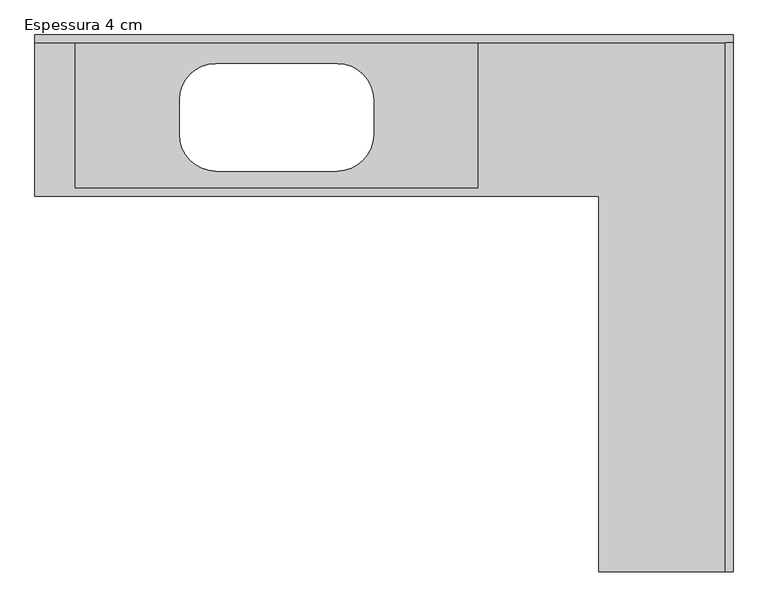
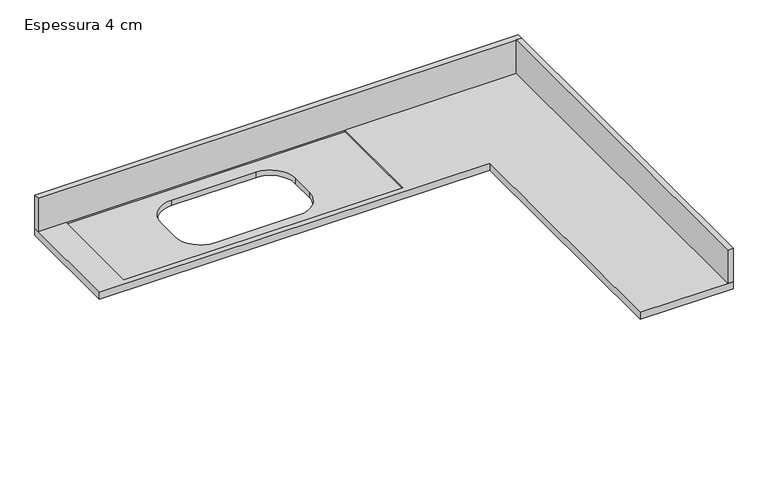
"""IFC4 building model written with IfcOpenShell, lengths in millimetres: furniture geometry, .BANCADA EM L_COZINHA_CUBA DUPLA : Espessura 4 cm."""

from ifc_helpers import new_model, si_unit, frame, origin, place, context, project, spatial, polyline, circle_curve, outline, extrude, source, transform, mapped, element, save
from ifc_brep_helpers import plane_surface, revolved_surface, advanced_brep


def espessura_4_cm_24cf57e0(model_context):
    return source(origin(), model_context, "Body", "SolidModel", [
        extrude(outline(polyline([(-30.0, -30.0), (0.0, -30.0), (0.0, -2000.0), (-30.0, -2000.0), (-30.0, -30.0)])), frame((0.0, 0.0, 900.0), z_axis=(0.0, 0.0, 1.0), x_axis=(1.0, 0.0, 0.0)), (0.0, 0.0, 1.0), 190.0),
        extrude(outline(polyline([(-2600.0, -30.0), (-2600.0, 0.0), (0.0, 0.0), (0.0, -30.0), (-2600.0, -30.0)])), frame((0.0, 0.0, 900.0), z_axis=(0.0, 0.0, 1.0), x_axis=(1.0, 0.0, 0.0)), (0.0, 0.0, 1.0), 190.0),
        advanced_brep(
        [(-500.0, -600.0, 860.0), (-2600.0, -600.0, 860.0), (-2600.0, 0.0, 860.0), (0.0, 0.0, 860.0), (0.0, -2000.0, 860.0), (-500.0, -2000.0, 860.0), (-1926.0, -107.0, 860.0), (-2061.0, -242.0, 860.0), (-2061.0, -372.0, 860.0), (-1926.0, -507.0, 860.0), (-1474.0, -507.0, 860.0), (-1339.0, -372.0, 860.0), (-1339.0, -242.0, 860.0), (-1474.0, -107.0, 860.0), (-500.0, -600.0, 900.0), (-500.0, -2000.0, 900.0), (0.0, -2000.0, 900.0), (0.0, 0.0, 900.0), (-2600.0, 0.0, 900.0), (-2600.0, -600.0, 900.0), (-950.0, -30.0, 900.0), (-950.0, -570.0, 900.0), (-2450.0, -570.0, 900.0), (-2450.0, -30.0, 900.0), (-1474.0, -107.0, 890.0), (-1926.0, -107.0, 890.0), (-1339.0, -242.0, 890.0), (-1339.0, -372.0, 890.0), (-1474.0, -507.0, 890.0), (-1926.0, -507.0, 890.0), (-2061.0, -372.0, 890.0), (-2061.0, -242.0, 890.0), (-950.0, -570.0, 890.0), (-950.0, -30.0, 890.0), (-2450.0, -30.0, 890.0), (-2450.0, -570.0, 890.0)],
        [
            (0, 1),
            (1, 2),
            (2, 3),
            (3, 4),
            (4, 5),
            (5, 0),
            (6, 7, circle_curve(frame((-1926.0, -242.0, 860.0), z_axis=(0.0, 0.0, 1.0), x_axis=(-1.0, 0.0, 0.0)), 135.0)),
            (7, 8),
            (8, 9, circle_curve(frame((-1926.0, -372.0, 860.0), z_axis=(0.0, 0.0, 1.0), x_axis=(-1.0, 0.0, 0.0)), 135.0)),
            (9, 10),
            (10, 11, circle_curve(frame((-1474.0, -372.0, 860.0), z_axis=(0.0, 0.0, 1.0), x_axis=(-1.0, 0.0, 0.0)), 135.0)),
            (11, 12),
            (12, 13, circle_curve(frame((-1474.0, -242.0, 860.0), z_axis=(0.0, 0.0, 1.0), x_axis=(-1.0, 0.0, 0.0)), 135.0)),
            (13, 6),
            (14, 15),
            (15, 16),
            (16, 17),
            (17, 18),
            (18, 19),
            (19, 14),
            (20, 21),
            (21, 22),
            (22, 23),
            (23, 20),
            (5, 15),
            (14, 0),
            (4, 16),
            (3, 17),
            (2, 18),
            (1, 19),
            (13, 24),
            (24, 25),
            (25, 6),
            (12, 26),
            (26, 24, circle_curve(frame((-1474.0, -242.0, 890.0), z_axis=(0.0, 0.0, 1.0), x_axis=(-1.0, 0.0, 0.0)), 135.0)),
            (11, 27),
            (27, 26),
            (10, 28),
            (28, 27, circle_curve(frame((-1474.0, -372.0, 890.0), z_axis=(0.0, 0.0, 1.0), x_axis=(-1.0, 0.0, 0.0)), 135.0)),
            (9, 29),
            (29, 28),
            (8, 30),
            (30, 29, circle_curve(frame((-1926.0, -372.0, 890.0), z_axis=(0.0, 0.0, 1.0), x_axis=(-1.0, 0.0, 0.0)), 135.0)),
            (7, 31),
            (31, 30),
            (25, 31, circle_curve(frame((-1926.0, -242.0, 890.0), z_axis=(0.0, 0.0, 1.0), x_axis=(-1.0, 0.0, 0.0)), 135.0)),
            (32, 33),
            (33, 34),
            (34, 35),
            (35, 32),
            (32, 21),
            (20, 33),
            (23, 34),
            (22, 35),
        ],
        [
            plane_surface(frame((-500.0, -600.0, 860.0), z_axis=(0.0, 0.0, -1.0), x_axis=(0.0, 1.0, 0.0))),
            plane_surface(frame((-500.0, -600.0, 900.0), z_axis=(0.0, 0.0, 1.0), x_axis=(0.0, -1.0, 0.0))),
            plane_surface(frame((-500.0, -600.0, 900.0), z_axis=(-1.0, 0.0, 0.0), x_axis=(0.0, 0.0, -1.0))),
            plane_surface(frame((-500.0, -2000.0, 900.0), z_axis=(0.0, -1.0, 0.0), x_axis=(0.0, 0.0, -1.0))),
            plane_surface(frame((0.0, -2000.0, 900.0), z_axis=(1.0, 0.0, 0.0), x_axis=(0.0, 0.0, -1.0))),
            plane_surface(frame((0.0, 0.0, 900.0), z_axis=(0.0, 1.0, 0.0), x_axis=(0.0, 0.0, -1.0))),
            plane_surface(frame((-2600.0, 0.0, 900.0), z_axis=(-1.0, 0.0, 0.0), x_axis=(0.0, 0.0, -1.0))),
            plane_surface(frame((-2600.0, -600.0, 900.0), z_axis=(0.0, -1.0, 0.0), x_axis=(0.0, 0.0, -1.0))),
            plane_surface(frame((-1926.0, -107.0, 900.0), z_axis=(0.0, -1.0, 0.0), x_axis=(0.0, 0.0, -1.0))),
            revolved_surface(polyline([(-1609.0, -242.0, 860.0), (-1609.0, -242.0, 890.0)]), (-1474.0, -242.0, 890.0), (0.0, 0.0, -1.0)),
            plane_surface(frame((-1339.0, -242.0, 900.0), z_axis=(-1.0, 0.0, 0.0), x_axis=(0.0, 0.0, -1.0))),
            revolved_surface(polyline([(-1609.0, -372.0, 860.0), (-1609.0, -372.0, 890.0)]), (-1474.0, -372.0, 890.0), (0.0, 0.0, -1.0)),
            plane_surface(frame((-1474.0, -507.0, 900.0), z_axis=(0.0, 1.0, 0.0), x_axis=(0.0, 0.0, -1.0))),
            revolved_surface(polyline([(-2061.0, -372.0, 860.0), (-2061.0, -372.0, 890.0)]), (-1926.0, -372.0, 890.0), (0.0, 0.0, -1.0)),
            plane_surface(frame((-2061.0, -372.0, 900.0), z_axis=(1.0, 0.0, 0.0), x_axis=(0.0, 0.0, -1.0))),
            revolved_surface(polyline([(-2061.0, -242.0, 860.0), (-2061.0, -242.0, 890.0)]), (-1926.0, -242.0, 890.0), (0.0, 0.0, -1.0)),
            plane_surface(frame((-950.0, -30.0, 890.0), z_axis=(0.0, 0.0, 1.0), x_axis=(0.0, -1.0, 0.0))),
            plane_surface(frame((-950.0, -570.0, 940.0), z_axis=(-1.0, 0.0, 0.0), x_axis=(0.0, 0.0, -1.0))),
            plane_surface(frame((-950.0, -30.0, 940.0), z_axis=(0.0, -1.0, 0.0), x_axis=(0.0, 0.0, -1.0))),
            plane_surface(frame((-2450.0, -30.0, 940.0), z_axis=(1.0, 0.0, 0.0), x_axis=(0.0, 0.0, -1.0))),
            plane_surface(frame((-2450.0, -570.0, 940.0), z_axis=(0.0, 1.0, 0.0), x_axis=(0.0, 0.0, -1.0))),
        ],
        [
            (0, [[1, 2, 3, 4, 5, 6], [7, 8, 9, 10, 11, 12, 13, 14]]),
            (1, [[15, 16, 17, 18, 19, 20], [21, 22, 23, 24]]),
            (2, [[-6, 25, -15, 26]]),
            (3, [[-5, 27, -16, -25]]),
            (4, [[-4, 28, -17, -27]]),
            (5, [[-3, 29, -18, -28]]),
            (6, [[-2, 30, -19, -29]]),
            (7, [[-1, -26, -20, -30]]),
            (8, [[-14, 31, 32, 33]]),
            (9, [[-13, 34, 35, -31]]),
            (10, [[-12, 36, 37, -34]]),
            (11, [[-11, 38, 39, -36]]),
            (12, [[-10, 40, 41, -38]]),
            (13, [[-9, 42, 43, -40]]),
            (14, [[-8, 44, 45, -42]]),
            (15, [[-7, -33, 46, -44]]),
            (16, [[47, 48, 49, 50], [-32, -35, -37, -39, -41, -43, -45, -46]]),
            (17, [[-47, 51, -21, 52]]),
            (18, [[-48, -52, -24, 53]]),
            (19, [[-49, -53, -23, 54]]),
            (20, [[-50, -54, -22, -51]]),
        ],
    ),
    ])


if __name__ == "__main__":
    model = new_model("IFC4")
    model_context = context("Model", 3, world=origin())
    ifc_project = project(units=[si_unit("LENGTHUNIT", "METRE", prefix="MILLI")], contexts=[model_context])
    site = spatial("IfcSite", under=ifc_project)
    building = spatial("IfcBuilding", under=site)
    placement = place(None, origin())
    espessura_4_cm_shape = espessura_4_cm_24cf57e0(model_context)
    element("IfcFurniture", 1, ObjectType=".BANCADA EM L_COZINHA_CUBA DUPLA : Espessura 4 cm", at=placement, inside=building, context=model_context, shape_type="MappedRepresentation", body=[
        mapped(espessura_4_cm_shape, transform((0.0, 0.0, 0.0), x_axis=(1.0, 0.0, 0.0), y_axis=(0.0, 1.0, 0.0), z_axis=(0.0, 0.0, 1.0))),
    ])
    save(model, "model.ifc")

# Revit data of these elements
# Type ".BANCADA EM L_COZINHA_CUBA DUPLA : Espessura 4 cm"
#   Offset esq área molhada [instance default] = 0.80 m
#   Largura área molhada [instance default] = 1.50 m
#   Largura principal [instance default] = 0.60 m
#   Largura da extensão [instance default] = 0.50 m
#   Espessura total da bancada [instance default] = 0.04 m
#   Espessura do frontão [instance default] = 0.03 m
#   Dist. cuba - borda [instance default] = 0.07 m
#   Compr. total principal [instance default] = 3.95 m
#   Compr. principal [instance default] = 3.45 m
#   Compr. total extensão [instance default] = 1.50 m
#   Compr. extensão [instance default] = 0.90 m
#   Altura do rebaixo da área molhada [instance default] = 0.01 m
#   Altura do frontão [instance default] = 0.20 m
#   Altura da bancada [instance default] = 0.90 m
#   Frontão fundos principal [instance default] = yes
#   Frontão fundos extensão [instance default] = yes
#   Frontão esquerdo principal [instance default] = yes
#   Frontão direito extensão [instance default] = yes
#   Material da bancada [instance default] = none
#   Default Elevation = 0
# Element 1 (IfcFurniture, ".BANCADA EM L_COZINHA_CUBA DUPLA : Espessura 4 cm")
#   Offset esq área molhada = 0.15 m
#   Compr. total principal = 2.60 m
#   Compr. principal = 2.10 m
#   Compr. total extensão = 2.00 m
#   Compr. extensão = 1.40 m
#   Frontão esquerdo principal = no
#   Frontão direito extensão = no
